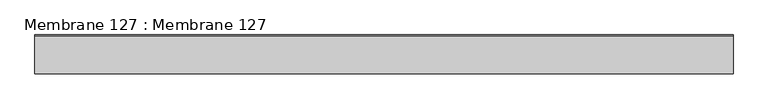
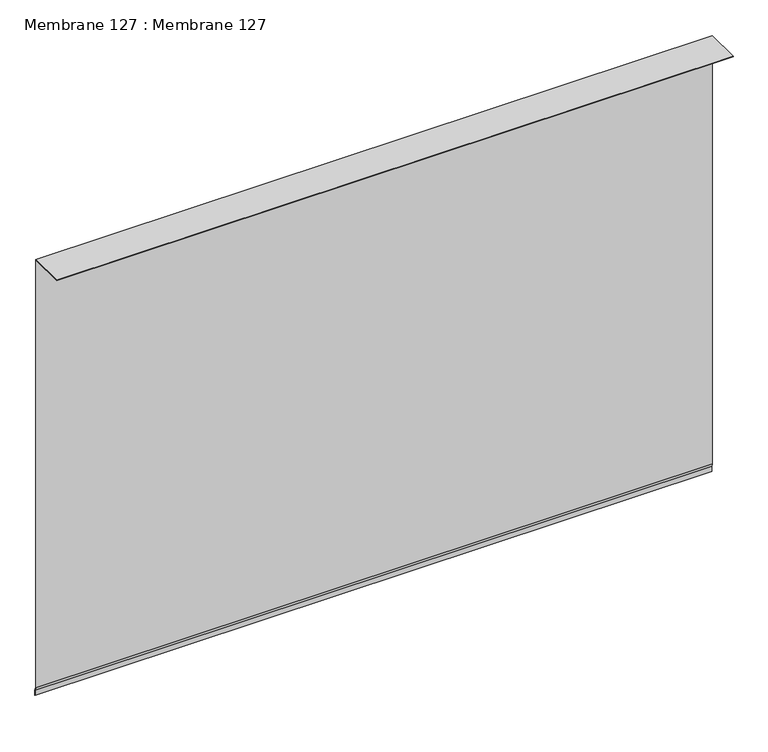
"""IFC4 building model written with IfcOpenShell, lengths in millimetres: proxy geometry, Membrane 127 : Membrane 127."""

from ifc_helpers import new_model, si_unit, frame, origin, place, context, project, spatial, polyline, outline, extrude, source, transform, mapped, element, save


def membrane_127_membrane_127_7833c3fc(model_context):
    return source(origin(), model_context, "Body", "SweptSolid", [
        extrude(outline(polyline([(10332.3117604, 40775.4101563), (10439.111229, 40775.4101563), (10439.111229, 39437.1078269), (10443.1968914, 39425.8825617), (10443.1968914, 39410.30025), (10442.1968914, 39410.30025), (10442.1968914, 39425.7062347), (10438.111229, 39436.9314999), (10438.111229, 40774.4101563), (10332.3117604, 40774.4101563), (10332.3117604, 40775.4101563)])), frame((3694.2883192, 0.0, 0.0), z_axis=(1.0, 0.0, 0.0), x_axis=(0.0, 1.0, 0.0)), (0.0, 0.0, 1.0), 2000.0),
    ])


if __name__ == "__main__":
    model = new_model("IFC4")
    model_context = context("Model", 3, world=origin())
    ifc_project = project(units=[si_unit("LENGTHUNIT", "METRE", prefix="MILLI")], contexts=[model_context])
    site = spatial("IfcSite", under=ifc_project)
    building = spatial("IfcBuilding", under=site)
    placement = place(None, origin())
    membrane_127_membrane_127_shape = membrane_127_membrane_127_7833c3fc(model_context)
    element("IfcBuildingElementProxy", 1, Name="Membrane 127 : Membrane 127", ObjectType="Membrane 127 : Membrane 127", at=placement, inside=building, context=model_context, shape_type="MappedRepresentation", body=[
        mapped(membrane_127_membrane_127_shape, transform((0.0, 0.0, 0.0), x_axis=(1.0, 0.0, 0.0), y_axis=(0.0, 1.0, 0.0), z_axis=(0.0, 0.0, 1.0))),
    ])
    save(model, "model.ifc")

# Revit data of these elements
# Type "Membrane 127 : Membrane 127"
#   NameOverride = "Membrane"
# Element 1 (IfcBuildingElementProxy, "Membrane 127 : Membrane 127")
#   Materials on its faces: "2 LAYERS NO. 30 ASTM D226 ASPHALT SATURATED ORGANIC FELT"
# Materials
#   "2 LAYERS NO. 30 ASTM D226 ASPHALT SATURATED ORGANIC FELT": class "Unassigned", colour RGB 46 171 0, transparency 0
